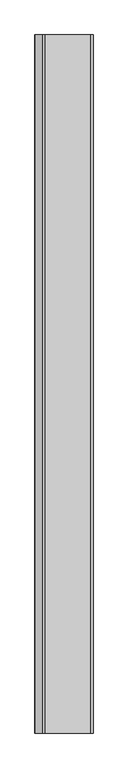
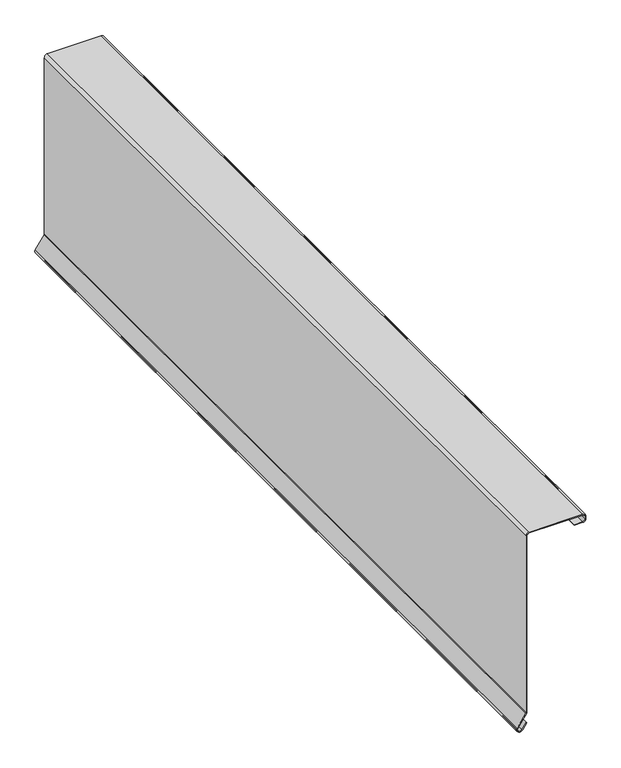
"""IFC4 building model written with IfcOpenShell, lengths in millimetres: proxy geometry, Flashing008 1279 : Flashing008 1279."""

from ifc_helpers import new_model, si_unit, point, frame, frame_2d, origin, place, context, project, spatial, polyline, circle_curve, trimmed, segment, composite_curve, outline, extrude, source, transform, mapped, element, save


def generic_models_516c5e6e(model_context):
    return source(origin(), model_context, "Body", "SweptSolid", [
        extrude(outline(composite_curve([segment(trimmed(circle_curve(frame_2d((43033.8898747, -6514.9327408)), 5.08), [point((43030.9678143, -6510.7772669))], [point((43029.7783694, -6517.9163501))], True, "CARTESIAN"), True, "CONTINUOUS"), segment(polyline([(43029.7783694, -6517.9163501), (43031.0710485, -6519.6977016)]), True, "CONTINUOUS"), segment(trimmed(circle_curve(frame_2d((43035.1825538, -6516.7140923)), 5.08), [point((43031.0710485, -6519.6977016))], [point((43038.0896432, -6520.8800533))], True, "CARTESIAN"), True, "CONTINUOUS"), segment(polyline([(43038.0896432, -6520.8800533), (43068.3424938, -6499.7690195)]), True, "CONTINUOUS"), segment(trimmed(circle_curve(frame_2d((43071.2495833, -6503.9349805)), 5.08), [point((43068.3424938, -6499.7690195))], [point((43071.2495833, -6498.8549805))], False, "CARTESIAN"), True, "CONTINUOUS"), segment(polyline([(43071.2495833, -6498.8549805), (43518.4785937, -6498.8549805)]), True, "CONTINUOUS"), segment(trimmed(circle_curve(frame_2d((43518.4785937, -6493.7749805)), 5.08), [point((43518.4785937, -6498.8549805))], [point((43523.5585937, -6493.7749805))], True, "CARTESIAN"), True, "CONTINUOUS"), segment(polyline([(43523.5585937, -6493.7749805), (43523.5585937, -6364.4349805)]), True, "CONTINUOUS"), segment(trimmed(circle_curve(frame_2d((43518.4785937, -6364.4349805)), 5.08), [point((43523.5585937, -6364.4349805))], [point((43518.4785937, -6359.3549805))], True, "CARTESIAN"), True, "CONTINUOUS"), segment(polyline([(43518.4785937, -6359.3549805), (43512.0721875, -6359.3549805)]), True, "CONTINUOUS"), segment(trimmed(circle_curve(frame_2d((43512.0721875, -6364.4349805)), 5.08), [point((43512.0721875, -6359.3549805))], [point((43506.9921875, -6364.4349805))], True, "CARTESIAN"), True, "CONTINUOUS"), segment(polyline([(43506.9921875, -6364.4349805), (43506.9921875, -6385.7314453), (43504.9921875, -6385.7314453), (43504.9921875, -6364.4349805)]), True, "CONTINUOUS"), segment(trimmed(circle_curve(frame_2d((43512.0721875, -6364.4349805)), 7.08), [point((43504.9921875, -6364.4349805))], [point((43512.0721875, -6357.3549805))], False, "CARTESIAN"), True, "CONTINUOUS"), segment(polyline([(43512.0721875, -6357.3549805), (43518.4785937, -6357.3549805)]), True, "CONTINUOUS"), segment(trimmed(circle_curve(frame_2d((43518.4785937, -6364.4349805)), 7.08), [point((43518.4785937, -6357.3549805))], [point((43525.5585937, -6364.4349805))], False, "CARTESIAN"), True, "CONTINUOUS"), segment(polyline([(43525.5585937, -6364.4349805), (43525.5585937, -6493.7749805)]), True, "CONTINUOUS"), segment(trimmed(circle_curve(frame_2d((43518.4785937, -6493.7749805)), 7.08), [point((43525.5585937, -6493.7749805))], [point((43518.4785937, -6500.8549805))], False, "CARTESIAN"), True, "CONTINUOUS"), segment(polyline([(43518.4785937, -6500.8549805), (43071.2495833, -6500.8549805)]), True, "CONTINUOUS"), segment(trimmed(circle_curve(frame_2d((43071.2495833, -6503.9349805)), 3.08), [point((43071.2495833, -6500.8549805))], [point((43069.4870172, -6501.4091616))], True, "CARTESIAN"), True, "CONTINUOUS"), segment(polyline([(43069.4870172, -6501.4091616), (43039.2341666, -6522.5201954)]), True, "CONTINUOUS"), segment(trimmed(circle_curve(frame_2d((43035.1825538, -6516.7140923)), 7.08), [point((43039.2341666, -6522.5201954))], [point((43029.4523457, -6520.872351))], False, "CARTESIAN"), True, "CONTINUOUS"), segment(polyline([(43029.4523457, -6520.872351), (43028.1596666, -6519.0909995)]), True, "CONTINUOUS"), segment(trimmed(circle_curve(frame_2d((43033.8898747, -6514.9327408)), 7.08), [point((43028.1596666, -6519.0909995))], [point((43029.8173969, -6509.1412536))], False, "CARTESIAN"), True, "CONTINUOUS"), segment(polyline([(43029.8173969, -6509.1412536), (43044.40427, -6498.8840062), (43045.5546875, -6500.5200195), (43030.9678143, -6510.7772669)]), True, "CONTINUOUS")], self_intersect=False)), frame((0.0, 7982.1531721, 0.0), z_axis=(0.0, 1.0, 0.0), x_axis=(0.0, 0.0, 1.0)), (0.0, 0.0, 1.0), 2000.0),
    ])


if __name__ == "__main__":
    model = new_model("IFC4")
    model_context = context("Model", 3, world=origin())
    ifc_project = project(units=[si_unit("LENGTHUNIT", "METRE", prefix="MILLI")], contexts=[model_context])
    site = spatial("IfcSite", under=ifc_project)
    building = spatial("IfcBuilding", under=site)
    placement = place(None, origin())
    generic_models_shape = generic_models_516c5e6e(model_context)
    element("IfcBuildingElementProxy", 1, Name="Flashing008 1279 : Flashing008 1279", ObjectType="Flashing008 1279 : Flashing008 1279", at=placement, inside=building, context=model_context, shape_type="MappedRepresentation", body=[
        mapped(generic_models_shape, transform((0.0, 0.0, 0.0), x_axis=(1.0, 0.0, 0.0), y_axis=(0.0, 1.0, 0.0), z_axis=(0.0, 0.0, 1.0))),
    ])
    save(model, "model.ifc")

# Revit data of these elements
# Type "Flashing008 1279 : Flashing008 1279"
#   NameOverride = "Flashing008"
# Element 1 (IfcBuildingElementProxy, "Flashing008 1279 : Flashing008 1279")
#   Materials on its faces: "HIGH EAVE FLASHING"
# Materials
#   "HIGH EAVE FLASHING": class "Unassigned", colour RGB 128 128 128, transparency 0
